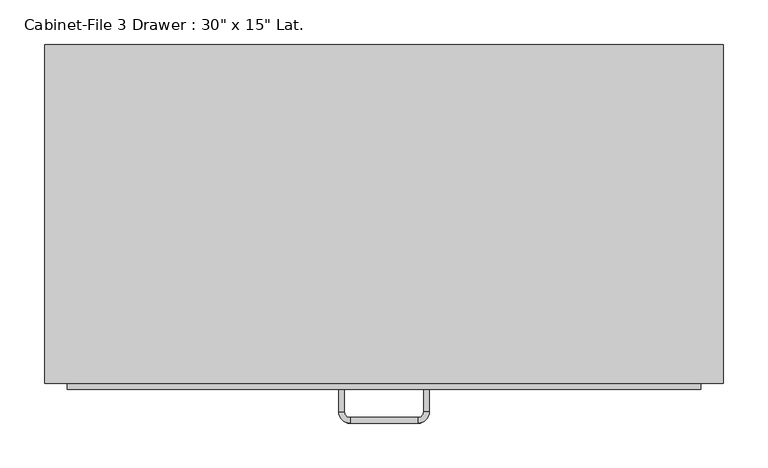
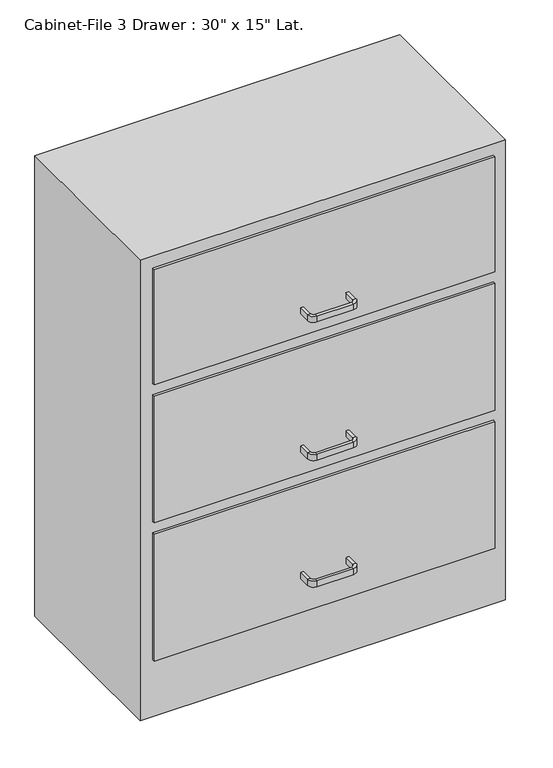
"""IFC4 building model written with IfcOpenShell, lengths in millimetres: furniture geometry."""

from ifc_helpers import new_model, si_unit, frame, origin, origin_with_axes, place, context, project, spatial, polyline, circle_curve, outline, extrude, source, transform, mapped, element, save
from ifc_brep_helpers import plane_surface, cylinder_surface, revolved_surface, advanced_brep


def furniture_4ebe9c9a(model_context):
    return source(origin(), model_context, "Body", "SolidModel", [
        extrude(outline(polyline([(253.103553, 48.3656999), (253.103553, -332.6343001), (-508.896447, -332.6343001), (-508.896447, 48.3656999), (253.103553, 48.3656999)])), origin_with_axes(), (0.0, 0.0, 1.0), 1016.0),
        extrude(outline(polyline([(227.703553, -338.9843001), (-483.496447, -338.9843001), (-483.496447, -332.6343001), (227.703553, -332.6343001), (227.703553, -338.9843001)])), frame((0.0, 0.0, 736.6), z_axis=(0.0, 0.0, 1.0), x_axis=(1.0, 0.0, 0.0)), (0.0, 0.0, 1.0), 254.0),
        extrude(outline(polyline([(227.703553, -338.9843001), (-483.496447, -338.9843001), (-483.496447, -332.6343001), (227.703553, -332.6343001), (227.703553, -338.9843001)])), frame((0.0, 0.0, 431.8), z_axis=(0.0, 0.0, 1.0), x_axis=(1.0, 0.0, 0.0)), (0.0, 0.0, 1.0), 279.4),
        extrude(outline(polyline([(227.703553, -338.9843001), (-483.496447, -338.9843001), (-483.496447, -332.6343001), (227.703553, -332.6343001), (227.703553, -338.9843001)])), frame((0.0, 0.0, 127.0), z_axis=(0.0, 0.0, 1.0), x_axis=(1.0, 0.0, 0.0)), (0.0, 0.0, 1.0), 279.4),
        advanced_brep(
        [(-172.346447, -338.9843001, 203.2), (-178.696447, -338.9843001, 203.2), (-178.696447, -338.9843001, 215.9), (-172.346447, -338.9843001, 215.9), (-172.346447, -364.3843001, 203.2), (-178.696447, -364.3843001, 203.2), (-178.696447, -364.3843001, 215.9), (-172.346447, -364.3843001, 215.9), (-165.996447, -377.0843001, 203.2), (-165.996447, -370.7343001, 203.2), (-165.996447, -377.0843001, 215.9), (-165.996447, -370.7343001, 215.9), (-89.796447, -370.7343001, 203.2), (-89.796447, -377.0843001, 203.2), (-89.796447, -377.0843001, 215.9), (-89.796447, -370.7343001, 215.9), (-77.096447, -364.3843001, 203.2), (-83.446447, -364.3843001, 203.2), (-77.096447, -364.3843001, 215.9), (-83.446447, -364.3843001, 215.9), (-83.446447, -338.9843001, 203.2), (-83.446447, -338.9843001, 215.9), (-77.096447, -338.9843001, 215.9), (-77.096447, -338.9843001, 203.2)],
        [
            (0, 1),
            (1, 2),
            (2, 3),
            (3, 0),
            (0, 4),
            (4, 5),
            (5, 1),
            (5, 6),
            (6, 2),
            (6, 7),
            (7, 3),
            (7, 4),
            (8, 5, circle_curve(frame((-165.996447, -364.3843001, 203.2), z_axis=(0.0, 0.0, -1.0), x_axis=(-1.0, 0.0, 0.0)), 12.7)),
            (4, 9, circle_curve(frame((-165.996447, -364.3843001, 203.2), z_axis=(0.0, 0.0, 1.0), x_axis=(-1.0, 0.0, 0.0)), 6.35)),
            (9, 8),
            (10, 6, circle_curve(frame((-165.996447, -364.3843001, 215.9), z_axis=(0.0, 0.0, -1.0), x_axis=(-1.0, 0.0, 0.0)), 12.7)),
            (8, 10),
            (11, 7, circle_curve(frame((-165.996447, -364.3843001, 215.9), z_axis=(0.0, 0.0, -1.0), x_axis=(-1.0, 0.0, 0.0)), 6.35)),
            (10, 11),
            (11, 9),
            (9, 12),
            (12, 13),
            (13, 8),
            (13, 14),
            (14, 10),
            (14, 15),
            (15, 11),
            (15, 12),
            (16, 13, circle_curve(frame((-89.796447, -364.3843001, 203.2), z_axis=(0.0, 0.0, -1.0), x_axis=(0.0, -1.0, 0.0)), 12.7)),
            (12, 17, circle_curve(frame((-89.796447, -364.3843001, 203.2), z_axis=(0.0, 0.0, 1.0), x_axis=(0.0, -1.0, 0.0)), 6.35)),
            (17, 16),
            (18, 14, circle_curve(frame((-89.796447, -364.3843001, 215.9), z_axis=(0.0, 0.0, -1.0), x_axis=(0.0, -1.0, 0.0)), 12.7)),
            (16, 18),
            (19, 15, circle_curve(frame((-89.796447, -364.3843001, 215.9), z_axis=(0.0, 0.0, -1.0), x_axis=(0.0, -1.0, 0.0)), 6.35)),
            (18, 19),
            (19, 17),
            (20, 21),
            (21, 22),
            (22, 23),
            (23, 20),
            (17, 20),
            (23, 16),
            (22, 18),
            (21, 19),
        ],
        [
            plane_surface(frame((-978.8216451, -338.9843001, 0.0), z_axis=(0.0, 1.0, 0.0), x_axis=(0.0, 0.0, -1.0))),
            plane_surface(frame((-172.346447, -338.9843001, 203.2), z_axis=(0.0, 0.0, -1.0), x_axis=(0.0, -1.0, 0.0))),
            plane_surface(frame((-178.696447, -338.9843001, 203.2), z_axis=(-1.0, 0.0, 0.0), x_axis=(0.0, -1.0, 0.0))),
            plane_surface(frame((-178.696447, -338.9843001, 215.9), z_axis=(0.0, 0.0, 1.0), x_axis=(0.0, -1.0, 0.0))),
            plane_surface(frame((-172.346447, -338.9843001, 215.9), z_axis=(1.0, 0.0, 0.0), x_axis=(0.0, -1.0, 0.0))),
            plane_surface(frame((-165.996447, -364.3843001, 203.2), z_axis=(0.0, 0.0, -1.0), x_axis=(-1.0, 0.0, 0.0))),
            cylinder_surface(frame((-165.996447, -364.3843001, 0.0), z_axis=(0.0, 0.0, 1.0), x_axis=(-1.0, 0.0, 0.0)), 12.7),
            plane_surface(frame((-165.996447, -364.3843001, 215.9), z_axis=(0.0, 0.0, 1.0), x_axis=(-1.0, 0.0, 0.0))),
            revolved_surface(polyline([(-172.34644699999998, -364.3843001, 215.9), (-172.34644699999998, -364.3843001, 203.2)]), (-165.996447, -364.3843001, 0.0), (0.0, 0.0, 1.0)),
            plane_surface(frame((-165.996447, -370.7343001, 203.2), z_axis=(0.0, 0.0, -1.0), x_axis=(1.0, 0.0, 0.0))),
            plane_surface(frame((-165.996447, -377.0843001, 203.2), z_axis=(0.0, -1.0, 0.0), x_axis=(1.0, 0.0, 0.0))),
            plane_surface(frame((-165.996447, -377.0843001, 215.9), z_axis=(0.0, 0.0, 1.0), x_axis=(1.0, 0.0, 0.0))),
            plane_surface(frame((-165.996447, -370.7343001, 215.9), z_axis=(0.0, 1.0, 0.0), x_axis=(1.0, 0.0, 0.0))),
            plane_surface(frame((-89.796447, -364.3843001, 203.2), z_axis=(0.0, 0.0, -1.0), x_axis=(0.0, -1.0, 0.0))),
            cylinder_surface(frame((-89.796447, -364.3843001, 0.0), z_axis=(0.0, 0.0, 1.0), x_axis=(0.0, -1.0, 0.0)), 12.7),
            plane_surface(frame((-89.796447, -364.3843001, 215.9), z_axis=(0.0, 0.0, 1.0), x_axis=(0.0, -1.0, 0.0))),
            revolved_surface(polyline([(-89.796447, -370.73430010000004, 215.9), (-89.796447, -370.73430010000004, 203.2)]), (-89.796447, -364.3843001, 0.0), (0.0, 0.0, 1.0)),
            plane_surface(frame((-877.2216451, -338.9843001, 0.0), z_axis=(0.0, 1.0, 0.0), x_axis=(0.0, 0.0, 1.0))),
            plane_surface(frame((-83.446447, -364.3843001, 203.2), z_axis=(0.0, 0.0, -1.0), x_axis=(0.0, 1.0, 0.0))),
            plane_surface(frame((-77.096447, -364.3843001, 203.2), z_axis=(1.0, 0.0, 0.0), x_axis=(0.0, 1.0, 0.0))),
            plane_surface(frame((-77.096447, -364.3843001, 215.9), z_axis=(0.0, 0.0, 1.0), x_axis=(0.0, 1.0, 0.0))),
            plane_surface(frame((-83.446447, -364.3843001, 215.9), z_axis=(-1.0, 0.0, 0.0), x_axis=(0.0, 1.0, 0.0))),
        ],
        [
            (0, [[1, 2, 3, 4]]),
            (1, [[-1, 5, 6, 7]]),
            (2, [[-2, -7, 8, 9]]),
            (3, [[-3, -9, 10, 11]]),
            (4, [[-4, -11, 12, -5]]),
            (5, [[13, -6, 14, 15]]),
            (6, [[16, -8, -13, 17]]),
            (7, [[18, -10, -16, 19]]),
            (8, [[-14, -12, -18, 20]]),
            (9, [[-15, 21, 22, 23]]),
            (10, [[-17, -23, 24, 25]]),
            (11, [[-19, -25, 26, 27]]),
            (12, [[-20, -27, 28, -21]]),
            (13, [[29, -22, 30, 31]]),
            (14, [[32, -24, -29, 33]]),
            (15, [[34, -26, -32, 35]]),
            (16, [[-30, -28, -34, 36]]),
            (17, [[37, 38, 39, 40]]),
            (18, [[-31, 41, -40, 42]]),
            (19, [[-33, -42, -39, 43]]),
            (20, [[-35, -43, -38, 44]]),
            (21, [[-36, -44, -37, -41]]),
        ],
    ),
        advanced_brep(
        [(-172.346447, -338.9843001, 482.6), (-178.696447, -338.9843001, 482.6), (-178.696447, -338.9843001, 495.3), (-172.346447, -338.9843001, 495.3), (-172.346447, -364.3843001, 482.6), (-178.696447, -364.3843001, 482.6), (-178.696447, -364.3843001, 495.3), (-172.346447, -364.3843001, 495.3), (-165.996447, -377.0843001, 482.6), (-165.996447, -370.7343001, 482.6), (-165.996447, -377.0843001, 495.3), (-165.996447, -370.7343001, 495.3), (-89.796447, -370.7343001, 482.6), (-89.796447, -377.0843001, 482.6), (-89.796447, -377.0843001, 495.3), (-89.796447, -370.7343001, 495.3), (-77.096447, -364.3843001, 482.6), (-83.446447, -364.3843001, 482.6), (-77.096447, -364.3843001, 495.3), (-83.446447, -364.3843001, 495.3), (-83.446447, -338.9843001, 482.6), (-83.446447, -338.9843001, 495.3), (-77.096447, -338.9843001, 495.3), (-77.096447, -338.9843001, 482.6)],
        [
            (0, 1),
            (1, 2),
            (2, 3),
            (3, 0),
            (0, 4),
            (4, 5),
            (5, 1),
            (5, 6),
            (6, 2),
            (6, 7),
            (7, 3),
            (7, 4),
            (8, 5, circle_curve(frame((-165.996447, -364.3843001, 482.6), z_axis=(0.0, 0.0, -1.0), x_axis=(-1.0, 0.0, 0.0)), 12.7)),
            (4, 9, circle_curve(frame((-165.996447, -364.3843001, 482.6), z_axis=(0.0, 0.0, 1.0), x_axis=(-1.0, 0.0, 0.0)), 6.35)),
            (9, 8),
            (10, 6, circle_curve(frame((-165.996447, -364.3843001, 495.3), z_axis=(0.0, 0.0, -1.0), x_axis=(-1.0, 0.0, 0.0)), 12.7)),
            (8, 10),
            (11, 7, circle_curve(frame((-165.996447, -364.3843001, 495.3), z_axis=(0.0, 0.0, -1.0), x_axis=(-1.0, 0.0, 0.0)), 6.35)),
            (10, 11),
            (11, 9),
            (9, 12),
            (12, 13),
            (13, 8),
            (13, 14),
            (14, 10),
            (14, 15),
            (15, 11),
            (15, 12),
            (16, 13, circle_curve(frame((-89.796447, -364.3843001, 482.6), z_axis=(0.0, 0.0, -1.0), x_axis=(0.0, -1.0, 0.0)), 12.7)),
            (12, 17, circle_curve(frame((-89.796447, -364.3843001, 482.6), z_axis=(0.0, 0.0, 1.0), x_axis=(0.0, -1.0, 0.0)), 6.35)),
            (17, 16),
            (18, 14, circle_curve(frame((-89.796447, -364.3843001, 495.3), z_axis=(0.0, 0.0, -1.0), x_axis=(0.0, -1.0, 0.0)), 12.7)),
            (16, 18),
            (19, 15, circle_curve(frame((-89.796447, -364.3843001, 495.3), z_axis=(0.0, 0.0, -1.0), x_axis=(0.0, -1.0, 0.0)), 6.35)),
            (18, 19),
            (19, 17),
            (20, 21),
            (21, 22),
            (22, 23),
            (23, 20),
            (17, 20),
            (23, 16),
            (22, 18),
            (21, 19),
        ],
        [
            plane_surface(frame((-978.8216451, -338.9843001, 0.0), z_axis=(0.0, 1.0, 0.0), x_axis=(0.0, 0.0, -1.0))),
            plane_surface(frame((-172.346447, -338.9843001, 482.6), z_axis=(0.0, 0.0, -1.0), x_axis=(0.0, -1.0, 0.0))),
            plane_surface(frame((-178.696447, -338.9843001, 482.6), z_axis=(-1.0, 0.0, 0.0), x_axis=(0.0, -1.0, 0.0))),
            plane_surface(frame((-178.696447, -338.9843001, 495.3), z_axis=(0.0, 0.0, 1.0), x_axis=(0.0, -1.0, 0.0))),
            plane_surface(frame((-172.346447, -338.9843001, 495.3), z_axis=(1.0, 0.0, 0.0), x_axis=(0.0, -1.0, 0.0))),
            plane_surface(frame((-165.996447, -364.3843001, 482.6), z_axis=(0.0, 0.0, -1.0), x_axis=(-1.0, 0.0, 0.0))),
            cylinder_surface(frame((-165.996447, -364.3843001, 0.0), z_axis=(0.0, 0.0, 1.0), x_axis=(-1.0, 0.0, 0.0)), 12.7),
            plane_surface(frame((-165.996447, -364.3843001, 495.3), z_axis=(0.0, 0.0, 1.0), x_axis=(-1.0, 0.0, 0.0))),
            revolved_surface(polyline([(-172.34644699999998, -364.3843001, 495.3), (-172.34644699999998, -364.3843001, 482.6)]), (-165.996447, -364.3843001, 0.0), (0.0, 0.0, 1.0)),
            plane_surface(frame((-165.996447, -370.7343001, 482.6), z_axis=(0.0, 0.0, -1.0), x_axis=(1.0, 0.0, 0.0))),
            plane_surface(frame((-165.996447, -377.0843001, 482.6), z_axis=(0.0, -1.0, 0.0), x_axis=(1.0, 0.0, 0.0))),
            plane_surface(frame((-165.996447, -377.0843001, 495.3), z_axis=(0.0, 0.0, 1.0), x_axis=(1.0, 0.0, 0.0))),
            plane_surface(frame((-165.996447, -370.7343001, 495.3), z_axis=(0.0, 1.0, 0.0), x_axis=(1.0, 0.0, 0.0))),
            plane_surface(frame((-89.796447, -364.3843001, 482.6), z_axis=(0.0, 0.0, -1.0), x_axis=(0.0, -1.0, 0.0))),
            cylinder_surface(frame((-89.796447, -364.3843001, 0.0), z_axis=(0.0, 0.0, 1.0), x_axis=(0.0, -1.0, 0.0)), 12.7),
            plane_surface(frame((-89.796447, -364.3843001, 495.3), z_axis=(0.0, 0.0, 1.0), x_axis=(0.0, -1.0, 0.0))),
            revolved_surface(polyline([(-89.796447, -370.73430010000004, 495.3), (-89.796447, -370.73430010000004, 482.6)]), (-89.796447, -364.3843001, 0.0), (0.0, 0.0, 1.0)),
            plane_surface(frame((-877.2216451, -338.9843001, 0.0), z_axis=(0.0, 1.0, 0.0), x_axis=(0.0, 0.0, 1.0))),
            plane_surface(frame((-83.446447, -364.3843001, 482.6), z_axis=(0.0, 0.0, -1.0), x_axis=(0.0, 1.0, 0.0))),
            plane_surface(frame((-77.096447, -364.3843001, 482.6), z_axis=(1.0, 0.0, 0.0), x_axis=(0.0, 1.0, 0.0))),
            plane_surface(frame((-77.096447, -364.3843001, 495.3), z_axis=(0.0, 0.0, 1.0), x_axis=(0.0, 1.0, 0.0))),
            plane_surface(frame((-83.446447, -364.3843001, 495.3), z_axis=(-1.0, 0.0, 0.0), x_axis=(0.0, 1.0, 0.0))),
        ],
        [
            (0, [[1, 2, 3, 4]]),
            (1, [[-1, 5, 6, 7]]),
            (2, [[-2, -7, 8, 9]]),
            (3, [[-3, -9, 10, 11]]),
            (4, [[-4, -11, 12, -5]]),
            (5, [[13, -6, 14, 15]]),
            (6, [[16, -8, -13, 17]]),
            (7, [[18, -10, -16, 19]]),
            (8, [[-14, -12, -18, 20]]),
            (9, [[-15, 21, 22, 23]]),
            (10, [[-17, -23, 24, 25]]),
            (11, [[-19, -25, 26, 27]]),
            (12, [[-20, -27, 28, -21]]),
            (13, [[29, -22, 30, 31]]),
            (14, [[32, -24, -29, 33]]),
            (15, [[34, -26, -32, 35]]),
            (16, [[-30, -28, -34, 36]]),
            (17, [[37, 38, 39, 40]]),
            (18, [[-31, 41, -40, 42]]),
            (19, [[-33, -42, -39, 43]]),
            (20, [[-35, -43, -38, 44]]),
            (21, [[-36, -44, -37, -41]]),
        ],
    ),
        advanced_brep(
        [(-172.346447, -338.9843001, 787.4), (-178.696447, -338.9843001, 787.4), (-178.696447, -338.9843001, 800.1), (-172.346447, -338.9843001, 800.1), (-172.346447, -364.3843001, 787.4), (-178.696447, -364.3843001, 787.4), (-178.696447, -364.3843001, 800.1), (-172.346447, -364.3843001, 800.1), (-165.996447, -377.0843001, 787.4), (-165.996447, -370.7343001, 787.4), (-165.996447, -377.0843001, 800.1), (-165.996447, -370.7343001, 800.1), (-89.796447, -370.7343001, 787.4), (-89.796447, -377.0843001, 787.4), (-89.796447, -377.0843001, 800.1), (-89.796447, -370.7343001, 800.1), (-77.096447, -364.3843001, 787.4), (-83.446447, -364.3843001, 787.4), (-77.096447, -364.3843001, 800.1), (-83.446447, -364.3843001, 800.1), (-83.446447, -338.9843001, 787.4), (-83.446447, -338.9843001, 800.1), (-77.096447, -338.9843001, 800.1), (-77.096447, -338.9843001, 787.4)],
        [
            (0, 1),
            (1, 2),
            (2, 3),
            (3, 0),
            (0, 4),
            (4, 5),
            (5, 1),
            (5, 6),
            (6, 2),
            (6, 7),
            (7, 3),
            (7, 4),
            (8, 5, circle_curve(frame((-165.996447, -364.3843001, 787.4), z_axis=(0.0, 0.0, -1.0), x_axis=(-1.0, 0.0, 0.0)), 12.7)),
            (4, 9, circle_curve(frame((-165.996447, -364.3843001, 787.4), z_axis=(0.0, 0.0, 1.0), x_axis=(-1.0, 0.0, 0.0)), 6.35)),
            (9, 8),
            (10, 6, circle_curve(frame((-165.996447, -364.3843001, 800.1), z_axis=(0.0, 0.0, -1.0), x_axis=(-1.0, 0.0, 0.0)), 12.7)),
            (8, 10),
            (11, 7, circle_curve(frame((-165.996447, -364.3843001, 800.1), z_axis=(0.0, 0.0, -1.0), x_axis=(-1.0, 0.0, 0.0)), 6.35)),
            (10, 11),
            (11, 9),
            (9, 12),
            (12, 13),
            (13, 8),
            (13, 14),
            (14, 10),
            (14, 15),
            (15, 11),
            (15, 12),
            (16, 13, circle_curve(frame((-89.796447, -364.3843001, 787.4), z_axis=(0.0, 0.0, -1.0), x_axis=(0.0, -1.0, 0.0)), 12.7)),
            (12, 17, circle_curve(frame((-89.796447, -364.3843001, 787.4), z_axis=(0.0, 0.0, 1.0), x_axis=(0.0, -1.0, 0.0)), 6.35)),
            (17, 16),
            (18, 14, circle_curve(frame((-89.796447, -364.3843001, 800.1), z_axis=(0.0, 0.0, -1.0), x_axis=(0.0, -1.0, 0.0)), 12.7)),
            (16, 18),
            (19, 15, circle_curve(frame((-89.796447, -364.3843001, 800.1), z_axis=(0.0, 0.0, -1.0), x_axis=(0.0, -1.0, 0.0)), 6.35)),
            (18, 19),
            (19, 17),
            (20, 21),
            (21, 22),
            (22, 23),
            (23, 20),
            (17, 20),
            (23, 16),
            (22, 18),
            (21, 19),
        ],
        [
            plane_surface(frame((-978.8216451, -338.9843001, 0.0), z_axis=(0.0, 1.0, 0.0), x_axis=(0.0, 0.0, -1.0))),
            plane_surface(frame((-172.346447, -338.9843001, 787.4), z_axis=(0.0, 0.0, -1.0), x_axis=(0.0, -1.0, 0.0))),
            plane_surface(frame((-178.696447, -338.9843001, 787.4), z_axis=(-1.0, 0.0, 0.0), x_axis=(0.0, -1.0, 0.0))),
            plane_surface(frame((-178.696447, -338.9843001, 800.1), z_axis=(0.0, 0.0, 1.0), x_axis=(0.0, -1.0, 0.0))),
            plane_surface(frame((-172.346447, -338.9843001, 800.1), z_axis=(1.0, 0.0, 0.0), x_axis=(0.0, -1.0, 0.0))),
            plane_surface(frame((-165.996447, -364.3843001, 787.4), z_axis=(0.0, 0.0, -1.0), x_axis=(-1.0, 0.0, 0.0))),
            cylinder_surface(frame((-165.996447, -364.3843001, 0.0), z_axis=(0.0, 0.0, 1.0), x_axis=(-1.0, 0.0, 0.0)), 12.7),
            plane_surface(frame((-165.996447, -364.3843001, 800.1), z_axis=(0.0, 0.0, 1.0), x_axis=(-1.0, 0.0, 0.0))),
            revolved_surface(polyline([(-172.34644699999998, -364.3843001, 800.1), (-172.34644699999998, -364.3843001, 787.4)]), (-165.996447, -364.3843001, 0.0), (0.0, 0.0, 1.0)),
            plane_surface(frame((-165.996447, -370.7343001, 787.4), z_axis=(0.0, 0.0, -1.0), x_axis=(1.0, 0.0, 0.0))),
            plane_surface(frame((-165.996447, -377.0843001, 787.4), z_axis=(0.0, -1.0, 0.0), x_axis=(1.0, 0.0, 0.0))),
            plane_surface(frame((-165.996447, -377.0843001, 800.1), z_axis=(0.0, 0.0, 1.0), x_axis=(1.0, 0.0, 0.0))),
            plane_surface(frame((-165.996447, -370.7343001, 800.1), z_axis=(0.0, 1.0, 0.0), x_axis=(1.0, 0.0, 0.0))),
            plane_surface(frame((-89.796447, -364.3843001, 787.4), z_axis=(0.0, 0.0, -1.0), x_axis=(0.0, -1.0, 0.0))),
            cylinder_surface(frame((-89.796447, -364.3843001, 0.0), z_axis=(0.0, 0.0, 1.0), x_axis=(0.0, -1.0, 0.0)), 12.7),
            plane_surface(frame((-89.796447, -364.3843001, 800.1), z_axis=(0.0, 0.0, 1.0), x_axis=(0.0, -1.0, 0.0))),
            revolved_surface(polyline([(-89.796447, -370.73430010000004, 800.1), (-89.796447, -370.73430010000004, 787.4)]), (-89.796447, -364.3843001, 0.0), (0.0, 0.0, 1.0)),
            plane_surface(frame((-877.2216451, -338.9843001, 0.0), z_axis=(0.0, 1.0, 0.0), x_axis=(0.0, 0.0, 1.0))),
            plane_surface(frame((-83.446447, -364.3843001, 787.4), z_axis=(0.0, 0.0, -1.0), x_axis=(0.0, 1.0, 0.0))),
            plane_surface(frame((-77.096447, -364.3843001, 787.4), z_axis=(1.0, 0.0, 0.0), x_axis=(0.0, 1.0, 0.0))),
            plane_surface(frame((-77.096447, -364.3843001, 800.1), z_axis=(0.0, 0.0, 1.0), x_axis=(0.0, 1.0, 0.0))),
            plane_surface(frame((-83.446447, -364.3843001, 800.1), z_axis=(-1.0, 0.0, 0.0), x_axis=(0.0, 1.0, 0.0))),
        ],
        [
            (0, [[1, 2, 3, 4]]),
            (1, [[-1, 5, 6, 7]]),
            (2, [[-2, -7, 8, 9]]),
            (3, [[-3, -9, 10, 11]]),
            (4, [[-4, -11, 12, -5]]),
            (5, [[13, -6, 14, 15]]),
            (6, [[16, -8, -13, 17]]),
            (7, [[18, -10, -16, 19]]),
            (8, [[-14, -12, -18, 20]]),
            (9, [[-15, 21, 22, 23]]),
            (10, [[-17, -23, 24, 25]]),
            (11, [[-19, -25, 26, 27]]),
            (12, [[-20, -27, 28, -21]]),
            (13, [[29, -22, 30, 31]]),
            (14, [[32, -24, -29, 33]]),
            (15, [[34, -26, -32, 35]]),
            (16, [[-30, -28, -34, 36]]),
            (17, [[37, 38, 39, 40]]),
            (18, [[-31, 41, -40, 42]]),
            (19, [[-33, -42, -39, 43]]),
            (20, [[-35, -43, -38, 44]]),
            (21, [[-36, -44, -37, -41]]),
        ],
    ),
    ])


if __name__ == "__main__":
    model = new_model("IFC4")
    model_context = context("Model", 3, world=origin())
    ifc_project = project(units=[si_unit("LENGTHUNIT", "METRE", prefix="MILLI")], contexts=[model_context])
    site = spatial("IfcSite", under=ifc_project)
    building = spatial("IfcBuilding", under=site)
    placement = place(None, origin())
    furniture_shape = furniture_4ebe9c9a(model_context)
    element("IfcFurniture", 1, ObjectType="Cabinet-File 3 Drawer : 30\" x 15\" Lat.", at=placement, inside=building, context=model_context, shape_type="MappedRepresentation", body=[
        mapped(furniture_shape, transform((0.0, 0.0, 0.0), x_axis=(1.0, 0.0, 0.0), y_axis=(0.0, 1.0, 0.0), z_axis=(0.0, 0.0, 1.0))),
    ])
    save(model, "model.ifc")

# Revit data of these elements
# Type "Cabinet-File 3 Drawer : 30\" x 15\" Lat."
#   Assembly Code = "E2020200"
#   Depth = 1' - 3"
#   Height = 3' - 4"
#   Width = 2' - 6"
#   Cabinet Material = Steel, Paint Finish, Ivory, Glossy
#   Handle Material = Steel, Chrome Plated
#   Default Elevation = 0
# Element 1 (IfcFurniture, "Cabinet-File 3 Drawer : 30\" x 15\" Lat.")
#   Materials on its faces: "Steel, Chrome Plated", "Steel, Paint Finish, Ivory, Glossy"
# Materials
#   "Steel, Paint Finish, Ivory, Glossy": class "Metal", colour RGB 247 247 239, transparency 0, Description = "Steel, paint finish, ivory, glossy", Cost = 0
#   "Steel, Chrome Plated": class "Metal", colour RGB 17 17 17, transparency 0, Description = "Chromiuim plated steel", Cost = 0
